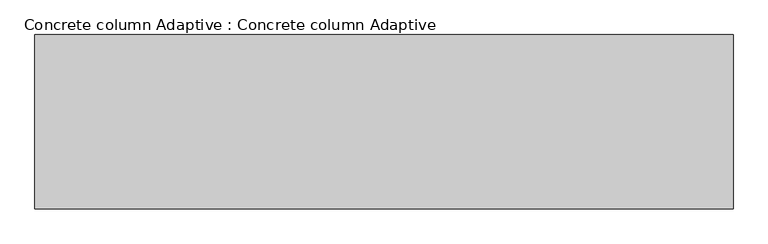
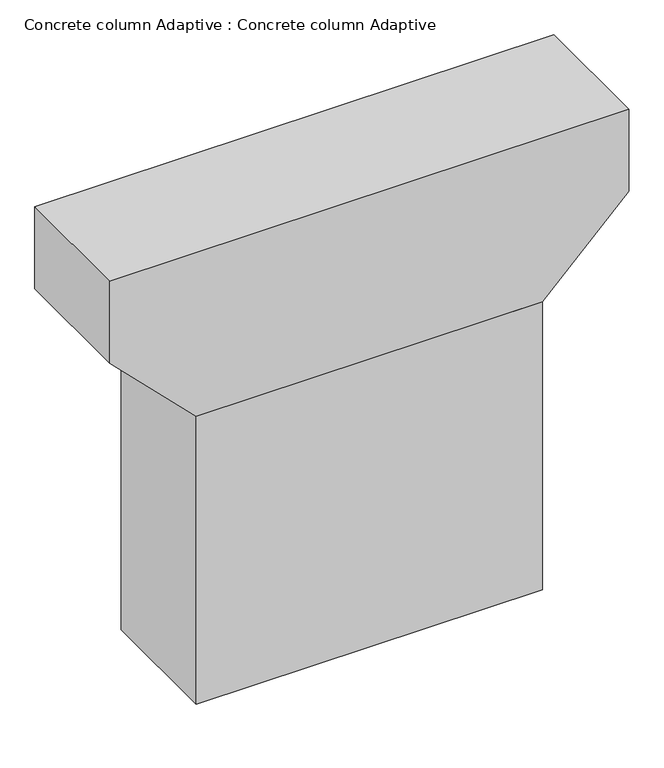
"""IFC4 building model written with IfcOpenShell, lengths in millimetres: proxy geometry, Concrete column Adaptive : Concrete column Adaptive."""

import ifcopenshell
import ifcopenshell.guid

model = None  # the IFC model being written
_history = None  # IfcOwnerHistory: only IFC2X3 demands one
_inside = {}  # id of a spatial element -> (the spatial element, [elements in it])
_under = {}  # id of a project, library or spatial element -> (it, [spatial elements below it])
_declared = {}  # id of a project -> (the project, [libraries it declares])
_typed = {}  # id of a type object -> (the type object, [elements of that type])
_made_of = {}  # id of a material, layer set ... -> (it, [elements and type objects made of it])


def new_model(schema):
    """Start an empty IFC model of exactly this schema.

    Asked for "IFC4X3", IfcOpenShell would pick the latest addendum, in which some entities
    have other attributes; the version numbers below select the first issue.
    IFC2X3 requires an IfcOwnerHistory on every rooted entity: one is made here for all.
    """
    global model, _history
    if schema == "IFC4X3":
        model = ifcopenshell.file(schema_version=(4, 3, 0, 0))
    else:
        model = ifcopenshell.file(schema=schema)
    _inside.clear()
    _under.clear()
    _declared.clear()
    _typed.clear()
    _made_of.clear()
    _history = None
    if model.schema == "IFC2X3":
        org = make("IfcOrganization", Name="unknown")
        user = make(
            "IfcPersonAndOrganization",
            ThePerson=make("IfcPerson", FamilyName="unknown"),
            TheOrganization=org,
        )
        app = make(
            "IfcApplication",
            ApplicationDeveloper=org,
            Version="unknown",
            ApplicationFullName="unknown",
            ApplicationIdentifier="unknown",
        )
        _history = make(
            "IfcOwnerHistory",
            OwningUser=user,
            OwningApplication=app,
            ChangeAction="ADDED",
            CreationDate=0,
        )
    return model


def make(cls, **values):
    """One entity of the class cls with the attributes given. An attribute that is None is left unset."""
    return model.create_entity(
        cls, **{name: value for name, value in values.items() if value is not None}
    )


def rooted(cls, **values):
    """An entity with a GlobalId (a new one), such as an element, a storey or a relation."""
    return make(cls, GlobalId=ifcopenshell.guid.new(), OwnerHistory=_history, **values)


def si_unit(unit_type, name, prefix=None):
    """IfcSIUnit, for example si_unit("LENGTHUNIT", "METRE", prefix="MILLI")."""
    return make("IfcSIUnit", UnitType=unit_type, Prefix=prefix, Name=name)


def assignment(units):
    """IfcUnitAssignment: the units of a project."""
    return None if units is None else make("IfcUnitAssignment", Units=units)


def point(xyz):
    """IfcCartesianPoint."""
    return None if xyz is None else make("IfcCartesianPoint", Coordinates=xyz)


def direction(xyz):
    """IfcDirection."""
    return None if xyz is None else make("IfcDirection", DirectionRatios=xyz)


def frame(location, z_axis=None, x_axis=None):
    """IfcAxis2Placement3D, a coordinate frame: its origin and axes. An axis left out is left unset."""
    return make(
        "IfcAxis2Placement3D",
        Location=point(location),
        Axis=direction(z_axis),
        RefDirection=direction(x_axis),
    )


def origin():
    """The frame at (0, 0, 0) with its axes left unset."""
    return frame((0.0, 0.0, 0.0))


def origin_with_axes():
    """The frame at (0, 0, 0) with the z axis (0, 0, 1) and the x axis (1, 0, 0) written out."""
    return frame((0.0, 0.0, 0.0), z_axis=(0.0, 0.0, 1.0), x_axis=(1.0, 0.0, 0.0))


def place(relative_to, where):
    """IfcLocalPlacement: puts the frame where relative to a parent placement (None: the world)."""
    return make(
        "IfcLocalPlacement", PlacementRelTo=relative_to, RelativePlacement=where
    )


def context(
    kind, dimensions, precision=None, world=None, true_north=None, identifier=None
):
    """IfcGeometricRepresentationContext, for example the 3D "Model" context."""
    return make(
        "IfcGeometricRepresentationContext",
        ContextIdentifier=identifier,
        ContextType=kind,
        CoordinateSpaceDimension=dimensions,
        Precision=precision,
        WorldCoordinateSystem=world,
        TrueNorth=true_north,
    )


def project(units=None, contexts=None):
    """IfcProject with its units and contexts."""
    return rooted(
        "IfcProject",
        Name="project",
        RepresentationContexts=contexts,
        UnitsInContext=assignment(units),
    )


def spatial(cls, under=None, at=None, **own):
    """A site, building, storey or space (cls), placed at a placement, below another one or the project."""
    s = rooted(cls, ObjectPlacement=at, **own)
    if under is not None:
        _under.setdefault(under.id(), (under, []))[1].append(s)
    return s


def polyline(points):
    """IfcPolyline through the points."""
    return make("IfcPolyline", Points=[point(p) for p in points])


def outline(outer, holes=None, kind="AREA"):
    """IfcArbitraryClosedProfileDef: a profile drawn as a closed curve; with holes, ...WithVoids."""
    if holes is None:
        return make("IfcArbitraryClosedProfileDef", ProfileType=kind, OuterCurve=outer)
    return make(
        "IfcArbitraryProfileDefWithVoids",
        ProfileType=kind,
        OuterCurve=outer,
        InnerCurves=holes,
    )


def extrude(swept, where, along, depth):
    """IfcExtrudedAreaSolid: the profile swept, set in the frame where, extruded along a direction by depth."""
    return make(
        "IfcExtrudedAreaSolid",
        SweptArea=swept,
        Position=where,
        ExtrudedDirection=direction(along),
        Depth=depth,
    )


def shape(context_of_items, identifier, shape_type, items):
    """IfcShapeRepresentation: the items that make up one representation, for example the "Body"."""
    return make(
        "IfcShapeRepresentation",
        ContextOfItems=context_of_items,
        RepresentationIdentifier=identifier,
        RepresentationType=shape_type,
        Items=items,
    )


def source(mapping_origin, context_of_items, identifier, shape_type, items):
    """IfcRepresentationMap: a shape defined once, which mapped items show again and again."""
    return make(
        "IfcRepresentationMap",
        MappingOrigin=mapping_origin,
        MappedRepresentation=shape(context_of_items, identifier, shape_type, items),
    )


def transform(
    local_origin,
    x_axis=None,
    y_axis=None,
    z_axis=None,
    scale=None,
    scale2=None,
    scale3=None,
    uniform=True,
):
    """IfcCartesianTransformationOperator3D, or its non-uniform kind. x_axis, y_axis, z_axis: its Axis1, 2, 3."""
    if uniform:
        return make(
            "IfcCartesianTransformationOperator3D",
            Axis1=direction(x_axis),
            Axis2=direction(y_axis),
            LocalOrigin=point(local_origin),
            Scale=scale,
            Axis3=direction(z_axis),
        )
    return make(
        "IfcCartesianTransformationOperator3DnonUniform",
        Axis1=direction(x_axis),
        Axis2=direction(y_axis),
        LocalOrigin=point(local_origin),
        Scale=scale,
        Axis3=direction(z_axis),
        Scale2=scale2,
        Scale3=scale3,
    )


def mapped(mapping_source, mapping_target):
    """IfcMappedItem: shows the shape of a source again, moved by a transform."""
    return make(
        "IfcMappedItem", MappingSource=mapping_source, MappingTarget=mapping_target
    )


def made_of(thing, what):
    """Note that an element or type object is made of a material, layer set ...; save() writes the relation."""
    if what is not None:
        _made_of.setdefault(what.id(), (what, []))[1].append(thing)
    return thing


def element(
    cls,
    number,
    at=None,
    inside=None,
    cuts=None,
    type_object=None,
    material=None,
    context=None,
    identifier="Body",
    shape_type=None,
    held_by="IfcProductDefinitionShape",
    body=None,
    shapes=None,
    **own,
):
    """One element of the class cls, such as IfcWall. Its Tag is "e" and its number.

    at: its placement. inside: the storey or other place that contains it. cuts: it is an
    opening in that element (IfcRelVoidsElement). A single representation is given by context,
    identifier, shape_type and body (its items); several are given by shapes. held_by: the class
    of the entity that holds the representations. save() writes the other relations.
    """
    e = rooted(cls, Tag="e%d" % number, ObjectPlacement=at, **own)
    if body is not None:
        shapes = [shape(context, identifier, shape_type, body)]
    if shapes is not None:
        e.Representation = make(held_by, Representations=shapes)
    if inside is not None:
        _inside.setdefault(inside.id(), (inside, []))[1].append(e)
    if cuts is not None:
        rooted(
            "IfcRelVoidsElement", RelatingBuildingElement=cuts, RelatedOpeningElement=e
        )
    if type_object is not None:
        _typed.setdefault(type_object.id(), (type_object, []))[1].append(e)
    return made_of(e, material)


def aggregate(whole, parts):
    """IfcRelAggregates: a whole, such as a stair, and the parts it consists of."""
    return rooted("IfcRelAggregates", RelatingObject=whole, RelatedObjects=parts)


def save(model, path):
    """Write the relations noted so far, then the file.

    IfcRelAggregates (storeys below a building ...), IfcRelContainedInSpatialStructure (elements
    in a storey), IfcRelDefinesByType, IfcRelAssociatesMaterial and IfcRelDeclares: one each for
    every whole, place, type object, material and project.
    """
    for whole, parts in _under.values():
        aggregate(whole, parts)
    for where, things in _inside.values():
        rooted(
            "IfcRelContainedInSpatialStructure",
            RelatedElements=things,
            RelatingStructure=where,
        )
    for kind, things in _typed.values():
        rooted("IfcRelDefinesByType", RelatedObjects=things, RelatingType=kind)
    for what, things in _made_of.values():
        rooted("IfcRelAssociatesMaterial", RelatedObjects=things, RelatingMaterial=what)
    for by, libraries in _declared.values():
        rooted("IfcRelDeclares", RelatingContext=by, RelatedDefinitions=libraries)
    model.write(path)


def concrete_column_adaptive_concrete_column_adaptive_77980e97(model_context):
    return source(origin(), model_context, "Body", "SweptSolid", [
        extrude(outline(polyline([(11034.0, 6000.0), (11034.0, -6000.0), (9034.0, -6000.0), (7034.0, -4000.0), (7034.0, 4000.0), (9034.0, 6000.0), (11034.0, 6000.0)])), frame((0.0, -1500.0, 0.0), z_axis=(0.0, 1.0, 0.0), x_axis=(0.0, 0.0, 1.0)), (0.0, 0.0, 1.0), 3000.0),
        extrude(outline(polyline([(-4000.0, -1500.0), (-4000.0, 1500.0), (4000.0, 1500.0), (4000.0, -1500.0), (-4000.0, -1500.0)])), origin_with_axes(), (0.0, 0.0, 1.0), 7034.0),
    ])


if __name__ == "__main__":
    model = new_model("IFC4")
    model_context = context("Model", 3, world=origin())
    ifc_project = project(units=[si_unit("LENGTHUNIT", "METRE", prefix="MILLI")], contexts=[model_context])
    site = spatial("IfcSite", under=ifc_project)
    building = spatial("IfcBuilding", under=site)
    placement = place(None, origin())
    concrete_column_adaptive_concrete_column_adaptive_shape = concrete_column_adaptive_concrete_column_adaptive_77980e97(model_context)
    element("IfcBuildingElementProxy", 1, Name="Concrete column Adaptive : Concrete column Adaptive", ObjectType="Concrete column Adaptive : Concrete column Adaptive", at=placement, inside=building, context=model_context, shape_type="MappedRepresentation", body=[
        mapped(concrete_column_adaptive_concrete_column_adaptive_shape, transform((0.0, 0.0, 0.0), x_axis=(1.0, 0.0, 0.0), y_axis=(0.0, 1.0, 0.0), z_axis=(0.0, 0.0, 1.0))),
    ])
    save(model, "model.ifc")

# Revit data of these elements
# Type "Concrete column Adaptive : Concrete column Adaptive"
#   Height [instance default] = 30000 mm
#   Default Elevation = 0
# Element 1 (IfcBuildingElementProxy, "Concrete column Adaptive : Concrete column Adaptive")
#   Height = 7034 mm
